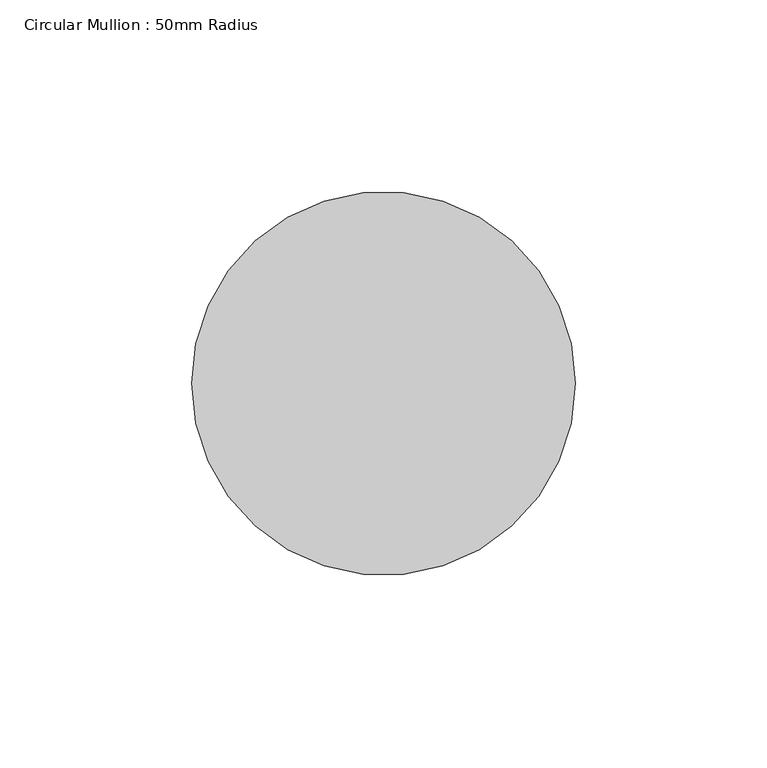
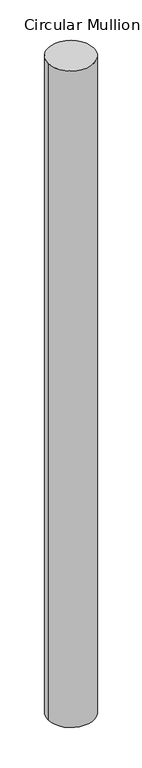
"""IFC4 building model written with IfcOpenShell, lengths in millimetres: member geometry, Circular Mullion : 50mm Radius."""

import ifcopenshell
import ifcopenshell.guid

model = None  # the IFC model being written
_history = None  # IfcOwnerHistory: only IFC2X3 demands one
_inside = {}  # id of a spatial element -> (the spatial element, [elements in it])
_under = {}  # id of a project, library or spatial element -> (it, [spatial elements below it])
_declared = {}  # id of a project -> (the project, [libraries it declares])
_typed = {}  # id of a type object -> (the type object, [elements of that type])
_made_of = {}  # id of a material, layer set ... -> (it, [elements and type objects made of it])


def new_model(schema):
    """Start an empty IFC model of exactly this schema.

    Asked for "IFC4X3", IfcOpenShell would pick the latest addendum, in which some entities
    have other attributes; the version numbers below select the first issue.
    IFC2X3 requires an IfcOwnerHistory on every rooted entity: one is made here for all.
    """
    global model, _history
    if schema == "IFC4X3":
        model = ifcopenshell.file(schema_version=(4, 3, 0, 0))
    else:
        model = ifcopenshell.file(schema=schema)
    _inside.clear()
    _under.clear()
    _declared.clear()
    _typed.clear()
    _made_of.clear()
    _history = None
    if model.schema == "IFC2X3":
        org = make("IfcOrganization", Name="unknown")
        user = make(
            "IfcPersonAndOrganization",
            ThePerson=make("IfcPerson", FamilyName="unknown"),
            TheOrganization=org,
        )
        app = make(
            "IfcApplication",
            ApplicationDeveloper=org,
            Version="unknown",
            ApplicationFullName="unknown",
            ApplicationIdentifier="unknown",
        )
        _history = make(
            "IfcOwnerHistory",
            OwningUser=user,
            OwningApplication=app,
            ChangeAction="ADDED",
            CreationDate=0,
        )
    return model


def make(cls, **values):
    """One entity of the class cls with the attributes given. An attribute that is None is left unset."""
    return model.create_entity(
        cls, **{name: value for name, value in values.items() if value is not None}
    )


def rooted(cls, **values):
    """An entity with a GlobalId (a new one), such as an element, a storey or a relation."""
    return make(cls, GlobalId=ifcopenshell.guid.new(), OwnerHistory=_history, **values)


def si_unit(unit_type, name, prefix=None):
    """IfcSIUnit, for example si_unit("LENGTHUNIT", "METRE", prefix="MILLI")."""
    return make("IfcSIUnit", UnitType=unit_type, Prefix=prefix, Name=name)


def assignment(units):
    """IfcUnitAssignment: the units of a project."""
    return None if units is None else make("IfcUnitAssignment", Units=units)


def point(xyz):
    """IfcCartesianPoint."""
    return None if xyz is None else make("IfcCartesianPoint", Coordinates=xyz)


def direction(xyz):
    """IfcDirection."""
    return None if xyz is None else make("IfcDirection", DirectionRatios=xyz)


def frame(location, z_axis=None, x_axis=None):
    """IfcAxis2Placement3D, a coordinate frame: its origin and axes. An axis left out is left unset."""
    return make(
        "IfcAxis2Placement3D",
        Location=point(location),
        Axis=direction(z_axis),
        RefDirection=direction(x_axis),
    )


def frame_2d(location, x_axis=None):
    """IfcAxis2Placement2D, a coordinate frame in the plane: its origin and x axis."""
    return make(
        "IfcAxis2Placement2D", Location=point(location), RefDirection=direction(x_axis)
    )


def origin():
    """The frame at (0, 0, 0) with its axes left unset."""
    return frame((0.0, 0.0, 0.0))


def origin_2d():
    """The frame at (0, 0) in the plane with its x axis left unset."""
    return frame_2d((0.0, 0.0))


def place(relative_to, where):
    """IfcLocalPlacement: puts the frame where relative to a parent placement (None: the world)."""
    return make(
        "IfcLocalPlacement", PlacementRelTo=relative_to, RelativePlacement=where
    )


def context(
    kind, dimensions, precision=None, world=None, true_north=None, identifier=None
):
    """IfcGeometricRepresentationContext, for example the 3D "Model" context."""
    return make(
        "IfcGeometricRepresentationContext",
        ContextIdentifier=identifier,
        ContextType=kind,
        CoordinateSpaceDimension=dimensions,
        Precision=precision,
        WorldCoordinateSystem=world,
        TrueNorth=true_north,
    )


def project(units=None, contexts=None):
    """IfcProject with its units and contexts."""
    return rooted(
        "IfcProject",
        Name="project",
        RepresentationContexts=contexts,
        UnitsInContext=assignment(units),
    )


def spatial(cls, under=None, at=None, **own):
    """A site, building, storey or space (cls), placed at a placement, below another one or the project."""
    s = rooted(cls, ObjectPlacement=at, **own)
    if under is not None:
        _under.setdefault(under.id(), (under, []))[1].append(s)
    return s


def circle_curve(where, radius):
    """IfcCircle in the frame where."""
    return make("IfcCircle", Position=where, Radius=radius)


def trimmed(basis, trim1, trim2, sense, master):
    """IfcTrimmedCurve: the piece of a basis curve between two trims."""
    return make(
        "IfcTrimmedCurve",
        BasisCurve=basis,
        Trim1=trim1,
        Trim2=trim2,
        SenseAgreement=sense,
        MasterRepresentation=master,
    )


def segment(curve, same_sense, transition):
    """IfcCompositeCurveSegment."""
    return make(
        "IfcCompositeCurveSegment",
        Transition=transition,
        SameSense=same_sense,
        ParentCurve=curve,
    )


def composite_curve(segments, self_intersect=None):
    """IfcCompositeCurve: segments joined end to end."""
    return make("IfcCompositeCurve", Segments=segments, SelfIntersect=self_intersect)


def outline(outer, holes=None, kind="AREA"):
    """IfcArbitraryClosedProfileDef: a profile drawn as a closed curve; with holes, ...WithVoids."""
    if holes is None:
        return make("IfcArbitraryClosedProfileDef", ProfileType=kind, OuterCurve=outer)
    return make(
        "IfcArbitraryProfileDefWithVoids",
        ProfileType=kind,
        OuterCurve=outer,
        InnerCurves=holes,
    )


def extrude(swept, where, along, depth):
    """IfcExtrudedAreaSolid: the profile swept, set in the frame where, extruded along a direction by depth."""
    return make(
        "IfcExtrudedAreaSolid",
        SweptArea=swept,
        Position=where,
        ExtrudedDirection=direction(along),
        Depth=depth,
    )


def shape(context_of_items, identifier, shape_type, items):
    """IfcShapeRepresentation: the items that make up one representation, for example the "Body"."""
    return make(
        "IfcShapeRepresentation",
        ContextOfItems=context_of_items,
        RepresentationIdentifier=identifier,
        RepresentationType=shape_type,
        Items=items,
    )


def source(mapping_origin, context_of_items, identifier, shape_type, items):
    """IfcRepresentationMap: a shape defined once, which mapped items show again and again."""
    return make(
        "IfcRepresentationMap",
        MappingOrigin=mapping_origin,
        MappedRepresentation=shape(context_of_items, identifier, shape_type, items),
    )


def transform(
    local_origin,
    x_axis=None,
    y_axis=None,
    z_axis=None,
    scale=None,
    scale2=None,
    scale3=None,
    uniform=True,
):
    """IfcCartesianTransformationOperator3D, or its non-uniform kind. x_axis, y_axis, z_axis: its Axis1, 2, 3."""
    if uniform:
        return make(
            "IfcCartesianTransformationOperator3D",
            Axis1=direction(x_axis),
            Axis2=direction(y_axis),
            LocalOrigin=point(local_origin),
            Scale=scale,
            Axis3=direction(z_axis),
        )
    return make(
        "IfcCartesianTransformationOperator3DnonUniform",
        Axis1=direction(x_axis),
        Axis2=direction(y_axis),
        LocalOrigin=point(local_origin),
        Scale=scale,
        Axis3=direction(z_axis),
        Scale2=scale2,
        Scale3=scale3,
    )


def mapped(mapping_source, mapping_target):
    """IfcMappedItem: shows the shape of a source again, moved by a transform."""
    return make(
        "IfcMappedItem", MappingSource=mapping_source, MappingTarget=mapping_target
    )


def made_of(thing, what):
    """Note that an element or type object is made of a material, layer set ...; save() writes the relation."""
    if what is not None:
        _made_of.setdefault(what.id(), (what, []))[1].append(thing)
    return thing


def element(
    cls,
    number,
    at=None,
    inside=None,
    cuts=None,
    type_object=None,
    material=None,
    context=None,
    identifier="Body",
    shape_type=None,
    held_by="IfcProductDefinitionShape",
    body=None,
    shapes=None,
    **own,
):
    """One element of the class cls, such as IfcWall. Its Tag is "e" and its number.

    at: its placement. inside: the storey or other place that contains it. cuts: it is an
    opening in that element (IfcRelVoidsElement). A single representation is given by context,
    identifier, shape_type and body (its items); several are given by shapes. held_by: the class
    of the entity that holds the representations. save() writes the other relations.
    """
    e = rooted(cls, Tag="e%d" % number, ObjectPlacement=at, **own)
    if body is not None:
        shapes = [shape(context, identifier, shape_type, body)]
    if shapes is not None:
        e.Representation = make(held_by, Representations=shapes)
    if inside is not None:
        _inside.setdefault(inside.id(), (inside, []))[1].append(e)
    if cuts is not None:
        rooted(
            "IfcRelVoidsElement", RelatingBuildingElement=cuts, RelatedOpeningElement=e
        )
    if type_object is not None:
        _typed.setdefault(type_object.id(), (type_object, []))[1].append(e)
    return made_of(e, material)


def aggregate(whole, parts):
    """IfcRelAggregates: a whole, such as a stair, and the parts it consists of."""
    return rooted("IfcRelAggregates", RelatingObject=whole, RelatedObjects=parts)


def save(model, path):
    """Write the relations noted so far, then the file.

    IfcRelAggregates (storeys below a building ...), IfcRelContainedInSpatialStructure (elements
    in a storey), IfcRelDefinesByType, IfcRelAssociatesMaterial and IfcRelDeclares: one each for
    every whole, place, type object, material and project.
    """
    for whole, parts in _under.values():
        aggregate(whole, parts)
    for where, things in _inside.values():
        rooted(
            "IfcRelContainedInSpatialStructure",
            RelatedElements=things,
            RelatingStructure=where,
        )
    for kind, things in _typed.values():
        rooted("IfcRelDefinesByType", RelatedObjects=things, RelatingType=kind)
    for what, things in _made_of.values():
        rooted("IfcRelAssociatesMaterial", RelatedObjects=things, RelatingMaterial=what)
    for by, libraries in _declared.values():
        rooted("IfcRelDeclares", RelatingContext=by, RelatedDefinitions=libraries)
    model.write(path)


def circular_mullion_50mm_radius_47164cad(model_context):
    return source(origin(), model_context, "Body", "SweptSolid", [
        extrude(outline(composite_curve([segment(trimmed(circle_curve(origin_2d(), 50.0), [point((50.0, 0.0))], [point((-50.0, 0.0))], False, "CARTESIAN"), True, "CONTINUOUS"), segment(trimmed(circle_curve(origin_2d(), 50.0), [point((-50.0, 0.0))], [point((50.0, 0.0))], False, "CARTESIAN"), True, "CONTINUOUS")], self_intersect=False)), frame((0.0, 0.0, -1510.5329928), z_axis=(0.0, 0.0, 1.0), x_axis=(1.0, 0.0, 0.0)), (0.0, 0.0, 1.0), 1510.5329928),
    ])


if __name__ == "__main__":
    model = new_model("IFC4")
    model_context = context("Model", 3, world=origin())
    ifc_project = project(units=[si_unit("LENGTHUNIT", "METRE", prefix="MILLI")], contexts=[model_context])
    site = spatial("IfcSite", under=ifc_project)
    building = spatial("IfcBuilding", under=site)
    placement = place(None, origin())
    circular_mullion_50mm_radius_shape = circular_mullion_50mm_radius_47164cad(model_context)
    element("IfcMember", 1, ObjectType="Circular Mullion : 50mm Radius", at=placement, inside=building, context=model_context, shape_type="MappedRepresentation", body=[
        mapped(circular_mullion_50mm_radius_shape, transform((0.0, 0.0, 0.0), x_axis=(1.0, 0.0, 0.0), y_axis=(0.0, 1.0, 0.0), z_axis=(0.0, 0.0, 1.0))),
    ])
    save(model, "model.ifc")

# Revit data of these elements
# Type "Circular Mullion : 50mm Radius"
#   built-in parameter 1007350 = 0.164042 (stored number, unit not read)
# Element 1 (IfcMember, "Circular Mullion : 50mm Radius")
#   Materials on its faces: "Aluminium"
# Materials
#   "Aluminium": class "Metal", colour RGB 247 247 247, transparency 0, Description = "Aluminium 6061", Cost = 0
